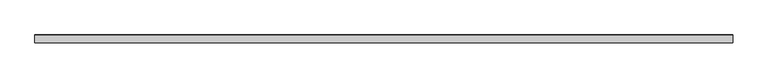
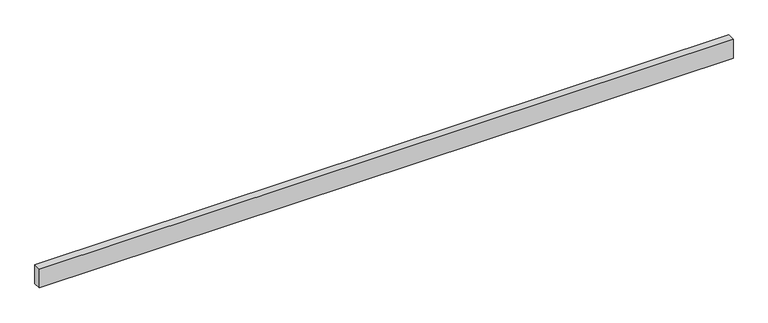
"""IFC4 building model written with IfcOpenShell, lengths in millimetres: proxy geometry, Generic Models 7:Generic Models 1:6:Generic Models 1:6 : Generic Models 7:Generic Models 1:337419:1 : Generic Models 7:Generic Models 1:6:Generic Models 1:6 : Generic Models 7:Generic Models 1:337419:312901."""

from ifc_helpers import new_model, si_unit, frame, origin, place, context, project, spatial, polyline, outline, extrude, source, transform, mapped, element, save


def generic_models_2fb7feb2(model_context):
    return source(origin(), model_context, "Body", "SweptSolid", [
        extrude(outline(polyline([(-579637.7301533, -24.8389136), (-579148.9271678, -14.6555181), (-579148.9271678, -84.5551275), (-579142.0790656, -84.5551275), (-579142.0790656, -1293.8930223), (-579637.7301533, -1293.8930223), (-579637.7301533, -24.8389136)])), frame((557809.7867239, 0.0, 0.0), z_axis=(1.0, 0.0, 0.0), x_axis=(0.0, 1.0, 0.0)), (0.0, 0.0, 1.0), 44500.8),
    ])


if __name__ == "__main__":
    model = new_model("IFC4")
    model_context = context("Model", 3, world=origin())
    ifc_project = project(units=[si_unit("LENGTHUNIT", "METRE", prefix="MILLI")], contexts=[model_context])
    site = spatial("IfcSite", under=ifc_project)
    building = spatial("IfcBuilding", under=site)
    placement = place(None, origin())
    generic_models_shape = generic_models_2fb7feb2(model_context)
    element("IfcBuildingElementProxy", 1, Name="Generic Models 7:Generic Models 1:6:Generic Models 1:6 : Generic Models 7:Generic Models 1:337419:1 : Generic Models 7:Generic Models 1:6:Generic Models 1:6 : Generic Models 7:Generic Models 1:337419:312901", ObjectType="Generic Models 7:Generic Models 1:6:Generic Models 1:6 : Generic Models 7:Generic Models 1:337419:1 : Generic Models 7:Generic Models 1:6:Generic Models 1:6 : Generic Models 7:Generic Models 1:337419:312901", at=placement, inside=building, context=model_context, shape_type="MappedRepresentation", body=[
        mapped(generic_models_shape, transform((0.0, 0.0, 0.0), x_axis=(1.0, 0.0, 0.0), y_axis=(0.0, 1.0, 0.0), z_axis=(0.0, 0.0, 1.0))),
    ])
    save(model, "model.ifc")

# Revit data of these elements
# Type "Generic Models 7:Generic Models 1:6:Generic Models 1:6 : Generic Models 7:Generic Models 1:337419:1 : Generic Models 7:Generic Models 1:6:Generic Models 1:6 : Generic Models 7:Generic Models 1:337419:312901"
#   NameOverride = "Generic Models 7:Generic Models 1:6:Generic Models 1:6 : Generic Models 7:Generic Models 1:337419:312901"
#   ObjectTypeOverride = "Generic Models 1:6 : Generic Models 7:Generic Models 1:337419"
#   Reference = "Generic Models 1"
#   Tag = "312901"
# Element 1 (IfcBuildingElementProxy, "Generic Models 7:Generic Models 1:6:Generic Models 1:6 : Generic Models 7:Generic Models 1:337419:1 : Generic Models 7:Generic Models 1:6:Generic Models 1:6 : Generic Models 7:Generic Models 1:337419:312901")
#   Materials on its faces: "GRADE"
# Materials
#   "GRADE": class "Generic", colour RGB 81 60 41, transparency 0, Description = "Soil", Cost = 0
